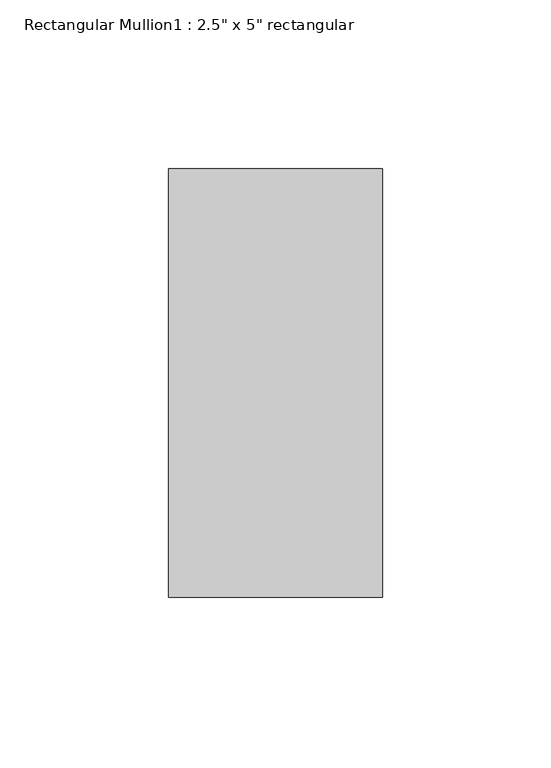
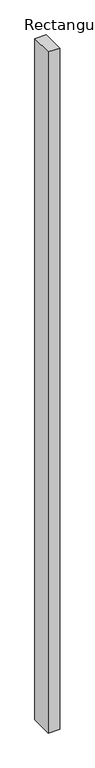
"""IFC4 building model written with IfcOpenShell, lengths in millimetres: member geometry."""

import ifcopenshell
import ifcopenshell.guid

model = None  # the IFC model being written
_history = None  # IfcOwnerHistory: only IFC2X3 demands one
_inside = {}  # id of a spatial element -> (the spatial element, [elements in it])
_under = {}  # id of a project, library or spatial element -> (it, [spatial elements below it])
_declared = {}  # id of a project -> (the project, [libraries it declares])
_typed = {}  # id of a type object -> (the type object, [elements of that type])
_made_of = {}  # id of a material, layer set ... -> (it, [elements and type objects made of it])


def new_model(schema):
    """Start an empty IFC model of exactly this schema.

    Asked for "IFC4X3", IfcOpenShell would pick the latest addendum, in which some entities
    have other attributes; the version numbers below select the first issue.
    IFC2X3 requires an IfcOwnerHistory on every rooted entity: one is made here for all.
    """
    global model, _history
    if schema == "IFC4X3":
        model = ifcopenshell.file(schema_version=(4, 3, 0, 0))
    else:
        model = ifcopenshell.file(schema=schema)
    _inside.clear()
    _under.clear()
    _declared.clear()
    _typed.clear()
    _made_of.clear()
    _history = None
    if model.schema == "IFC2X3":
        org = make("IfcOrganization", Name="unknown")
        user = make(
            "IfcPersonAndOrganization",
            ThePerson=make("IfcPerson", FamilyName="unknown"),
            TheOrganization=org,
        )
        app = make(
            "IfcApplication",
            ApplicationDeveloper=org,
            Version="unknown",
            ApplicationFullName="unknown",
            ApplicationIdentifier="unknown",
        )
        _history = make(
            "IfcOwnerHistory",
            OwningUser=user,
            OwningApplication=app,
            ChangeAction="ADDED",
            CreationDate=0,
        )
    return model


def make(cls, **values):
    """One entity of the class cls with the attributes given. An attribute that is None is left unset."""
    return model.create_entity(
        cls, **{name: value for name, value in values.items() if value is not None}
    )


def rooted(cls, **values):
    """An entity with a GlobalId (a new one), such as an element, a storey or a relation."""
    return make(cls, GlobalId=ifcopenshell.guid.new(), OwnerHistory=_history, **values)


def si_unit(unit_type, name, prefix=None):
    """IfcSIUnit, for example si_unit("LENGTHUNIT", "METRE", prefix="MILLI")."""
    return make("IfcSIUnit", UnitType=unit_type, Prefix=prefix, Name=name)


def assignment(units):
    """IfcUnitAssignment: the units of a project."""
    return None if units is None else make("IfcUnitAssignment", Units=units)


def point(xyz):
    """IfcCartesianPoint."""
    return None if xyz is None else make("IfcCartesianPoint", Coordinates=xyz)


def direction(xyz):
    """IfcDirection."""
    return None if xyz is None else make("IfcDirection", DirectionRatios=xyz)


def frame(location, z_axis=None, x_axis=None):
    """IfcAxis2Placement3D, a coordinate frame: its origin and axes. An axis left out is left unset."""
    return make(
        "IfcAxis2Placement3D",
        Location=point(location),
        Axis=direction(z_axis),
        RefDirection=direction(x_axis),
    )


def origin():
    """The frame at (0, 0, 0) with its axes left unset."""
    return frame((0.0, 0.0, 0.0))


def place(relative_to, where):
    """IfcLocalPlacement: puts the frame where relative to a parent placement (None: the world)."""
    return make(
        "IfcLocalPlacement", PlacementRelTo=relative_to, RelativePlacement=where
    )


def context(
    kind, dimensions, precision=None, world=None, true_north=None, identifier=None
):
    """IfcGeometricRepresentationContext, for example the 3D "Model" context."""
    return make(
        "IfcGeometricRepresentationContext",
        ContextIdentifier=identifier,
        ContextType=kind,
        CoordinateSpaceDimension=dimensions,
        Precision=precision,
        WorldCoordinateSystem=world,
        TrueNorth=true_north,
    )


def project(units=None, contexts=None):
    """IfcProject with its units and contexts."""
    return rooted(
        "IfcProject",
        Name="project",
        RepresentationContexts=contexts,
        UnitsInContext=assignment(units),
    )


def spatial(cls, under=None, at=None, **own):
    """A site, building, storey or space (cls), placed at a placement, below another one or the project."""
    s = rooted(cls, ObjectPlacement=at, **own)
    if under is not None:
        _under.setdefault(under.id(), (under, []))[1].append(s)
    return s


def polyline(points):
    """IfcPolyline through the points."""
    return make("IfcPolyline", Points=[point(p) for p in points])


def outline(outer, holes=None, kind="AREA"):
    """IfcArbitraryClosedProfileDef: a profile drawn as a closed curve; with holes, ...WithVoids."""
    if holes is None:
        return make("IfcArbitraryClosedProfileDef", ProfileType=kind, OuterCurve=outer)
    return make(
        "IfcArbitraryProfileDefWithVoids",
        ProfileType=kind,
        OuterCurve=outer,
        InnerCurves=holes,
    )


def extrude(swept, where, along, depth):
    """IfcExtrudedAreaSolid: the profile swept, set in the frame where, extruded along a direction by depth."""
    return make(
        "IfcExtrudedAreaSolid",
        SweptArea=swept,
        Position=where,
        ExtrudedDirection=direction(along),
        Depth=depth,
    )


def shape(context_of_items, identifier, shape_type, items):
    """IfcShapeRepresentation: the items that make up one representation, for example the "Body"."""
    return make(
        "IfcShapeRepresentation",
        ContextOfItems=context_of_items,
        RepresentationIdentifier=identifier,
        RepresentationType=shape_type,
        Items=items,
    )


def source(mapping_origin, context_of_items, identifier, shape_type, items):
    """IfcRepresentationMap: a shape defined once, which mapped items show again and again."""
    return make(
        "IfcRepresentationMap",
        MappingOrigin=mapping_origin,
        MappedRepresentation=shape(context_of_items, identifier, shape_type, items),
    )


def transform(
    local_origin,
    x_axis=None,
    y_axis=None,
    z_axis=None,
    scale=None,
    scale2=None,
    scale3=None,
    uniform=True,
):
    """IfcCartesianTransformationOperator3D, or its non-uniform kind. x_axis, y_axis, z_axis: its Axis1, 2, 3."""
    if uniform:
        return make(
            "IfcCartesianTransformationOperator3D",
            Axis1=direction(x_axis),
            Axis2=direction(y_axis),
            LocalOrigin=point(local_origin),
            Scale=scale,
            Axis3=direction(z_axis),
        )
    return make(
        "IfcCartesianTransformationOperator3DnonUniform",
        Axis1=direction(x_axis),
        Axis2=direction(y_axis),
        LocalOrigin=point(local_origin),
        Scale=scale,
        Axis3=direction(z_axis),
        Scale2=scale2,
        Scale3=scale3,
    )


def mapped(mapping_source, mapping_target):
    """IfcMappedItem: shows the shape of a source again, moved by a transform."""
    return make(
        "IfcMappedItem", MappingSource=mapping_source, MappingTarget=mapping_target
    )


def made_of(thing, what):
    """Note that an element or type object is made of a material, layer set ...; save() writes the relation."""
    if what is not None:
        _made_of.setdefault(what.id(), (what, []))[1].append(thing)
    return thing


def element(
    cls,
    number,
    at=None,
    inside=None,
    cuts=None,
    type_object=None,
    material=None,
    context=None,
    identifier="Body",
    shape_type=None,
    held_by="IfcProductDefinitionShape",
    body=None,
    shapes=None,
    **own,
):
    """One element of the class cls, such as IfcWall. Its Tag is "e" and its number.

    at: its placement. inside: the storey or other place that contains it. cuts: it is an
    opening in that element (IfcRelVoidsElement). A single representation is given by context,
    identifier, shape_type and body (its items); several are given by shapes. held_by: the class
    of the entity that holds the representations. save() writes the other relations.
    """
    e = rooted(cls, Tag="e%d" % number, ObjectPlacement=at, **own)
    if body is not None:
        shapes = [shape(context, identifier, shape_type, body)]
    if shapes is not None:
        e.Representation = make(held_by, Representations=shapes)
    if inside is not None:
        _inside.setdefault(inside.id(), (inside, []))[1].append(e)
    if cuts is not None:
        rooted(
            "IfcRelVoidsElement", RelatingBuildingElement=cuts, RelatedOpeningElement=e
        )
    if type_object is not None:
        _typed.setdefault(type_object.id(), (type_object, []))[1].append(e)
    return made_of(e, material)


def aggregate(whole, parts):
    """IfcRelAggregates: a whole, such as a stair, and the parts it consists of."""
    return rooted("IfcRelAggregates", RelatingObject=whole, RelatedObjects=parts)


def save(model, path):
    """Write the relations noted so far, then the file.

    IfcRelAggregates (storeys below a building ...), IfcRelContainedInSpatialStructure (elements
    in a storey), IfcRelDefinesByType, IfcRelAssociatesMaterial and IfcRelDeclares: one each for
    every whole, place, type object, material and project.
    """
    for whole, parts in _under.values():
        aggregate(whole, parts)
    for where, things in _inside.values():
        rooted(
            "IfcRelContainedInSpatialStructure",
            RelatedElements=things,
            RelatingStructure=where,
        )
    for kind, things in _typed.values():
        rooted("IfcRelDefinesByType", RelatedObjects=things, RelatingType=kind)
    for what, things in _made_of.values():
        rooted("IfcRelAssociatesMaterial", RelatedObjects=things, RelatingMaterial=what)
    for by, libraries in _declared.values():
        rooted("IfcRelDeclares", RelatingContext=by, RelatedDefinitions=libraries)
    model.write(path)


def member_01a33192(model_context):
    return source(origin(), model_context, "Body", "SweptSolid", [
        extrude(outline(polyline([(31.75, 63.5), (31.75, -63.5), (-31.75, -63.5), (-31.75, 63.5), (31.75, 63.5)])), frame((0.0, 0.0, -3971.7835741), z_axis=(0.0, 0.0, 1.0), x_axis=(1.0, 0.0, 0.0)), (0.0, 0.0, 1.0), 3971.7835741),
    ])


if __name__ == "__main__":
    model = new_model("IFC4")
    model_context = context("Model", 3, world=origin())
    ifc_project = project(units=[si_unit("LENGTHUNIT", "METRE", prefix="MILLI")], contexts=[model_context])
    site = spatial("IfcSite", under=ifc_project)
    building = spatial("IfcBuilding", under=site)
    placement = place(None, origin())
    member_shape = member_01a33192(model_context)
    element("IfcMember", 1, ObjectType="Rectangular Mullion1 : 2.5\" x 5\" rectangular", at=placement, inside=building, context=model_context, shape_type="MappedRepresentation", body=[
        mapped(member_shape, transform((0.0, 0.0, 0.0), x_axis=(1.0, 0.0, 0.0), y_axis=(0.0, 1.0, 0.0), z_axis=(0.0, 0.0, 1.0))),
    ])
    save(model, "model.ifc")

# Revit data of these elements
# Type "Rectangular Mullion1 : 2.5\" x 5\" rectangular"
#   built-in parameter 1007304 = 0.416667 (stored number, unit not read)
#   built-in parameter 1007301 = 0.104167 (stored number, unit not read)
#   built-in parameter 1007300 = 0.104167 (stored number, unit not read)
# Element 1 (IfcMember, "Rectangular Mullion1 : 2.5\" x 5\" rectangular")
#   Materials on its faces: "support-frame"
# Materials
#   "support-frame": class "Unassigned", colour RGB 233 233 233, transparency 0, Cost = 0
